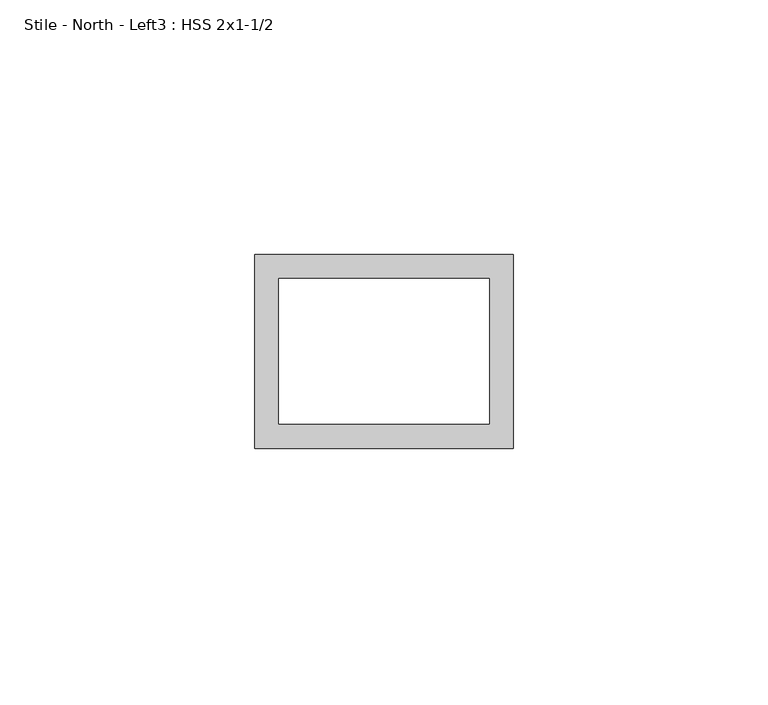
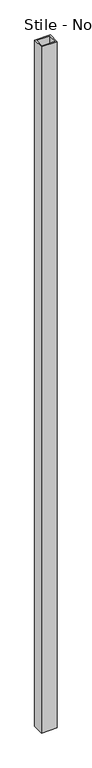
"""IFC4 building model written with IfcOpenShell, lengths in millimetres: proxy geometry, Stile - North - Left3 : HSS 2x1-1/2."""

from ifc_helpers import new_model, si_unit, frame, origin, place, context, project, spatial, polyline, outline, extrude, source, transform, mapped, element, save


def stile_north_left3_hss_2x1_1_2_870a2a95(model_context):
    return source(origin(), model_context, "Body", "SweptSolid", [
        extrude(outline(polyline([(587365.8934739, -534109.3663841), (587416.6934739, -534109.3663841), (587416.6934739, -534147.4663841), (587365.8934739, -534147.4663841), (587365.8934739, -534109.3663841)]), holes=[polyline([(587370.6559739, -534114.1288841), (587370.6559739, -534142.7038841), (587411.9309739, -534142.7038841), (587411.9309739, -534114.1288841), (587370.6559739, -534114.1288841)])]), frame((0.0, 0.0, 50.8), z_axis=(0.0, 0.0, 1.0), x_axis=(1.0, 0.0, 0.0)), (0.0, 0.0, 1.0), 2349.5),
    ])


if __name__ == "__main__":
    model = new_model("IFC4")
    model_context = context("Model", 3, world=origin())
    ifc_project = project(units=[si_unit("LENGTHUNIT", "METRE", prefix="MILLI")], contexts=[model_context])
    site = spatial("IfcSite", under=ifc_project)
    building = spatial("IfcBuilding", under=site)
    placement = place(None, origin())
    stile_north_left3_hss_2x1_1_2_shape = stile_north_left3_hss_2x1_1_2_870a2a95(model_context)
    element("IfcBuildingElementProxy", 1, Name="Stile - North - Left3 : HSS 2x1-1/2", ObjectType="Stile - North - Left3 : HSS 2x1-1/2", at=placement, inside=building, context=model_context, shape_type="MappedRepresentation", body=[
        mapped(stile_north_left3_hss_2x1_1_2_shape, transform((0.0, 0.0, 0.0), x_axis=(1.0, 0.0, 0.0), y_axis=(0.0, 1.0, 0.0), z_axis=(0.0, 0.0, 1.0))),
    ])
    save(model, "model.ifc")

# Revit data of these elements
# Element 1 (IfcBuildingElementProxy, "Stile - North - Left3 : HSS 2x1-1/2")
#   Materials on its faces: "1-1/2\"X2\" GALV. STL HSS TUBING"
# Materials
#   "1-1/2\"X2\" GALV. STL HSS TUBING": class "Generic", colour RGB 211 211 207, transparency 0, Cost = 0
